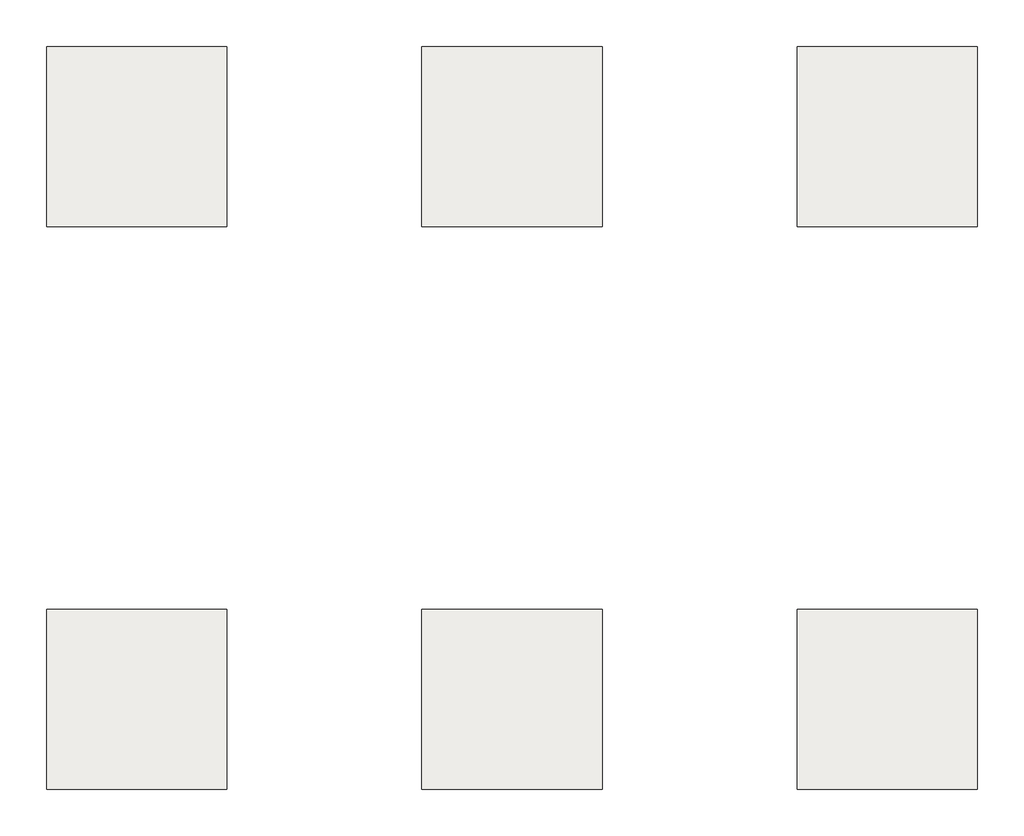
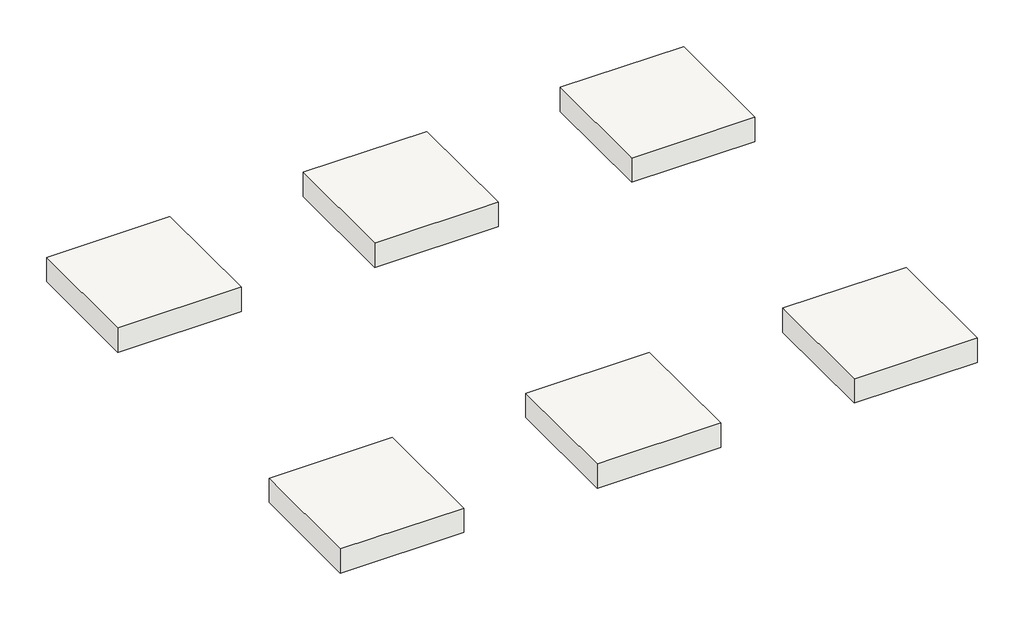
# Not in any storey: 6 slabs.
"""IFC4 building model written with IfcOpenShell, lengths in millimetres."""

import ifcopenshell
import ifcopenshell.guid

model = None  # the IFC model being written
_history = None  # IfcOwnerHistory: only IFC2X3 demands one
_inside = {}  # id of a spatial element -> (the spatial element, [elements in it])
_under = {}  # id of a project, library or spatial element -> (it, [spatial elements below it])
_declared = {}  # id of a project -> (the project, [libraries it declares])
_typed = {}  # id of a type object -> (the type object, [elements of that type])
_made_of = {}  # id of a material, layer set ... -> (it, [elements and type objects made of it])


def new_model(schema):
    """Start an empty IFC model of exactly this schema.

    Asked for "IFC4X3", IfcOpenShell would pick the latest addendum, in which some entities
    have other attributes; the version numbers below select the first issue.
    IFC2X3 requires an IfcOwnerHistory on every rooted entity: one is made here for all.
    """
    global model, _history
    if schema == "IFC4X3":
        model = ifcopenshell.file(schema_version=(4, 3, 0, 0))
    else:
        model = ifcopenshell.file(schema=schema)
    _inside.clear()
    _under.clear()
    _declared.clear()
    _typed.clear()
    _made_of.clear()
    _history = None
    if model.schema == "IFC2X3":
        org = make("IfcOrganization", Name="unknown")
        user = make(
            "IfcPersonAndOrganization",
            ThePerson=make("IfcPerson", FamilyName="unknown"),
            TheOrganization=org,
        )
        app = make(
            "IfcApplication",
            ApplicationDeveloper=org,
            Version="unknown",
            ApplicationFullName="unknown",
            ApplicationIdentifier="unknown",
        )
        _history = make(
            "IfcOwnerHistory",
            OwningUser=user,
            OwningApplication=app,
            ChangeAction="ADDED",
            CreationDate=0,
        )
    return model


def make(cls, **values):
    """One entity of the class cls with the attributes given. An attribute that is None is left unset."""
    return model.create_entity(
        cls, **{name: value for name, value in values.items() if value is not None}
    )


def rooted(cls, **values):
    """An entity with a GlobalId (a new one), such as an element, a storey or a relation."""
    return make(cls, GlobalId=ifcopenshell.guid.new(), OwnerHistory=_history, **values)


def si_unit(unit_type, name, prefix=None):
    """IfcSIUnit, for example si_unit("LENGTHUNIT", "METRE", prefix="MILLI")."""
    return make("IfcSIUnit", UnitType=unit_type, Prefix=prefix, Name=name)


def assignment(units):
    """IfcUnitAssignment: the units of a project."""
    return None if units is None else make("IfcUnitAssignment", Units=units)


def point(xyz):
    """IfcCartesianPoint."""
    return None if xyz is None else make("IfcCartesianPoint", Coordinates=xyz)


def direction(xyz):
    """IfcDirection."""
    return None if xyz is None else make("IfcDirection", DirectionRatios=xyz)


def frame(location, z_axis=None, x_axis=None):
    """IfcAxis2Placement3D, a coordinate frame: its origin and axes. An axis left out is left unset."""
    return make(
        "IfcAxis2Placement3D",
        Location=point(location),
        Axis=direction(z_axis),
        RefDirection=direction(x_axis),
    )


def origin():
    """The frame at (0, 0, 0) with its axes left unset."""
    return frame((0.0, 0.0, 0.0))


def place(relative_to, where):
    """IfcLocalPlacement: puts the frame where relative to a parent placement (None: the world)."""
    return make(
        "IfcLocalPlacement", PlacementRelTo=relative_to, RelativePlacement=where
    )


def context(
    kind, dimensions, precision=None, world=None, true_north=None, identifier=None
):
    """IfcGeometricRepresentationContext, for example the 3D "Model" context."""
    return make(
        "IfcGeometricRepresentationContext",
        ContextIdentifier=identifier,
        ContextType=kind,
        CoordinateSpaceDimension=dimensions,
        Precision=precision,
        WorldCoordinateSystem=world,
        TrueNorth=true_north,
    )


def project(units=None, contexts=None):
    """IfcProject with its units and contexts."""
    return rooted(
        "IfcProject",
        Name="project",
        RepresentationContexts=contexts,
        UnitsInContext=assignment(units),
    )


def spatial(cls, under=None, at=None, **own):
    """A site, building, storey or space (cls), placed at a placement, below another one or the project."""
    s = rooted(cls, ObjectPlacement=at, **own)
    if under is not None:
        _under.setdefault(under.id(), (under, []))[1].append(s)
    return s


def polyline(points):
    """IfcPolyline through the points."""
    return make("IfcPolyline", Points=[point(p) for p in points])


def outline(outer, holes=None, kind="AREA"):
    """IfcArbitraryClosedProfileDef: a profile drawn as a closed curve; with holes, ...WithVoids."""
    if holes is None:
        return make("IfcArbitraryClosedProfileDef", ProfileType=kind, OuterCurve=outer)
    return make(
        "IfcArbitraryProfileDefWithVoids",
        ProfileType=kind,
        OuterCurve=outer,
        InnerCurves=holes,
    )


def extrude(swept, where, along, depth):
    """IfcExtrudedAreaSolid: the profile swept, set in the frame where, extruded along a direction by depth."""
    return make(
        "IfcExtrudedAreaSolid",
        SweptArea=swept,
        Position=where,
        ExtrudedDirection=direction(along),
        Depth=depth,
    )


def shape(context_of_items, identifier, shape_type, items):
    """IfcShapeRepresentation: the items that make up one representation, for example the "Body"."""
    return make(
        "IfcShapeRepresentation",
        ContextOfItems=context_of_items,
        RepresentationIdentifier=identifier,
        RepresentationType=shape_type,
        Items=items,
    )


def source(mapping_origin, context_of_items, identifier, shape_type, items):
    """IfcRepresentationMap: a shape defined once, which mapped items show again and again."""
    return make(
        "IfcRepresentationMap",
        MappingOrigin=mapping_origin,
        MappedRepresentation=shape(context_of_items, identifier, shape_type, items),
    )


def transform(
    local_origin,
    x_axis=None,
    y_axis=None,
    z_axis=None,
    scale=None,
    scale2=None,
    scale3=None,
    uniform=True,
):
    """IfcCartesianTransformationOperator3D, or its non-uniform kind. x_axis, y_axis, z_axis: its Axis1, 2, 3."""
    if uniform:
        return make(
            "IfcCartesianTransformationOperator3D",
            Axis1=direction(x_axis),
            Axis2=direction(y_axis),
            LocalOrigin=point(local_origin),
            Scale=scale,
            Axis3=direction(z_axis),
        )
    return make(
        "IfcCartesianTransformationOperator3DnonUniform",
        Axis1=direction(x_axis),
        Axis2=direction(y_axis),
        LocalOrigin=point(local_origin),
        Scale=scale,
        Axis3=direction(z_axis),
        Scale2=scale2,
        Scale3=scale3,
    )


def mapped(mapping_source, mapping_target):
    """IfcMappedItem: shows the shape of a source again, moved by a transform."""
    return make(
        "IfcMappedItem", MappingSource=mapping_source, MappingTarget=mapping_target
    )


def made_of(thing, what):
    """Note that an element or type object is made of a material, layer set ...; save() writes the relation."""
    if what is not None:
        _made_of.setdefault(what.id(), (what, []))[1].append(thing)
    return thing


def element(
    cls,
    number,
    at=None,
    inside=None,
    cuts=None,
    type_object=None,
    material=None,
    context=None,
    identifier="Body",
    shape_type=None,
    held_by="IfcProductDefinitionShape",
    body=None,
    shapes=None,
    **own,
):
    """One element of the class cls, such as IfcWall. Its Tag is "e" and its number.

    at: its placement. inside: the storey or other place that contains it. cuts: it is an
    opening in that element (IfcRelVoidsElement). A single representation is given by context,
    identifier, shape_type and body (its items); several are given by shapes. held_by: the class
    of the entity that holds the representations. save() writes the other relations.
    """
    e = rooted(cls, Tag="e%d" % number, ObjectPlacement=at, **own)
    if body is not None:
        shapes = [shape(context, identifier, shape_type, body)]
    if shapes is not None:
        e.Representation = make(held_by, Representations=shapes)
    if inside is not None:
        _inside.setdefault(inside.id(), (inside, []))[1].append(e)
    if cuts is not None:
        rooted(
            "IfcRelVoidsElement", RelatingBuildingElement=cuts, RelatedOpeningElement=e
        )
    if type_object is not None:
        _typed.setdefault(type_object.id(), (type_object, []))[1].append(e)
    return made_of(e, material)


def aggregate(whole, parts):
    """IfcRelAggregates: a whole, such as a stair, and the parts it consists of."""
    return rooted("IfcRelAggregates", RelatingObject=whole, RelatedObjects=parts)


def save(model, path):
    """Write the relations noted so far, then the file.

    IfcRelAggregates (storeys below a building ...), IfcRelContainedInSpatialStructure (elements
    in a storey), IfcRelDefinesByType, IfcRelAssociatesMaterial and IfcRelDeclares: one each for
    every whole, place, type object, material and project.
    """
    for whole, parts in _under.values():
        aggregate(whole, parts)
    for where, things in _inside.values():
        rooted(
            "IfcRelContainedInSpatialStructure",
            RelatedElements=things,
            RelatingStructure=where,
        )
    for kind, things in _typed.values():
        rooted("IfcRelDefinesByType", RelatedObjects=things, RelatingType=kind)
    for what, things in _made_of.values():
        rooted("IfcRelAssociatesMaterial", RelatedObjects=things, RelatingMaterial=what)
    for by, libraries in _declared.values():
        rooted("IfcRelDeclares", RelatingContext=by, RelatedDefinitions=libraries)
    model.write(path)


def ft211_2400x2400x500_5fe39465(model_context):
    return source(origin(), model_context, "Body", "SweptSolid", [
        extrude(outline(polyline([(1200.0, 1200.0), (1200.0, -1200.0), (-1200.0, -1200.0), (-1200.0, 1200.0), (1200.0, 1200.0)])), frame((0.0, 0.0, -500.0), z_axis=(0.0, 0.0, 1.0), x_axis=(1.0, 0.0, 0.0)), (0.0, 0.0, 1.0), 500.0),
    ])


model = new_model("IFC4")

# Units and contexts
model_context = context("Model", 3, world=origin())
ifc_project = project(units=[si_unit("LENGTHUNIT", "METRE", prefix="MILLI")], contexts=[model_context])

# Site, building
site = spatial("IfcSite", under=ifc_project)
building = spatial("IfcBuilding", under=site)

# Slabs
placement = place(None, origin())
element("IfcSlab", 1, ObjectType="FT211-Footing-Rectangular_더미삭제 : FT211_2400x2400x500", at=placement, inside=building, context=model_context, shape_type="SweptSolid", body=[
    extrude(outline(polyline([(11200.0, 22199.5208589), (11200.0, 19799.5208589), (8800.0, 19799.5208589), (8800.0, 22199.5208589), (11200.0, 22199.5208589)])), frame((0.0, 0.0, -1800.0), z_axis=(0.0, 0.0, 1.0), x_axis=(1.0, 0.0, 0.0)), (0.0, 0.0, 1.0), 500.0),
])
element("IfcSlab", 2, ObjectType="FT211-Footing-Rectangular_더미삭제 : FT211_2400x2400x500", at=placement, inside=building, context=model_context, shape_type="SweptSolid", body=[
    extrude(outline(polyline([(6200.0, 22199.5208589), (6200.0, 19799.5208589), (3800.0, 19799.5208589), (3800.0, 22199.5208589), (6200.0, 22199.5208589)])), frame((0.0, 0.0, -1800.0), z_axis=(0.0, 0.0, 1.0), x_axis=(1.0, 0.0, 0.0)), (0.0, 0.0, 1.0), 500.0),
])
element("IfcSlab", 3, ObjectType="FT211-Footing-Rectangular_더미삭제 : FT211_2400x2400x500", at=placement, inside=building, context=model_context, shape_type="SweptSolid", body=[
    extrude(outline(polyline([(1200.0, 22199.5208589), (1200.0, 19799.5208589), (-1200.0, 19799.5208589), (-1200.0, 22199.5208589), (1200.0, 22199.5208589)])), frame((0.0, 0.0, -1800.0), z_axis=(0.0, 0.0, 1.0), x_axis=(1.0, 0.0, 0.0)), (0.0, 0.0, 1.0), 500.0),
])
element("IfcSlab", 4, ObjectType="FT211-Footing-Rectangular_더미삭제 : FT211_2400x2400x500", at=placement, inside=building, context=model_context, shape_type="SweptSolid", body=[
    extrude(outline(polyline([(1200.0, 14699.5208589), (1200.0, 12299.5208589), (-1200.0, 12299.5208589), (-1200.0, 14699.5208589), (1200.0, 14699.5208589)])), frame((0.0, 0.0, -1800.0), z_axis=(0.0, 0.0, 1.0), x_axis=(1.0, 0.0, 0.0)), (0.0, 0.0, 1.0), 500.0),
])
ft211_2400x2400x500_shape = ft211_2400x2400x500_5fe39465(model_context)
element("IfcSlab", 5, ObjectType="FT211-Footing-Rectangular_더미삭제 : FT211_2400x2400x500", at=placement, inside=building, context=model_context, shape_type="MappedRepresentation", body=[
    mapped(ft211_2400x2400x500_shape, transform((5000.0, 13499.5208589, -1300.0), x_axis=(1.0, 0.0, 0.0), y_axis=(0.0, 1.0, 0.0), z_axis=(0.0, 0.0, 1.0))),
])
element("IfcSlab", 6, ObjectType="FT211-Footing-Rectangular_더미삭제 : FT211_2400x2400x500", at=placement, inside=building, context=model_context, shape_type="MappedRepresentation", body=[
    mapped(ft211_2400x2400x500_shape, transform((10000.0, 13499.5208589, -1300.0), x_axis=(1.0, 0.0, 0.0), y_axis=(0.0, 1.0, 0.0), z_axis=(0.0, 0.0, 1.0))),
])

save(model, "model.ifc")

# Revit data of these elements
# Project information
#   Building Name = "MAIN GATE SECURITY BUILDING"
#   Project Status = "Project Status"
#   Client Name = "현대엔지니어링"
#   Project Address = "서울시 종로구 율곡로 75(계동)"
#   Project Name = "Therma Visayas Energy Project"
#   Project Number = "-"
# Grids (mm)
#   "A": line (0, 24502.793) -> (0, 11308.625)
#   "B": line (5000, 24502.793) -> (5000, 11308.625)
#   "C": line (10000, 24502.793) -> (10000, 11308.625)
#   "1": line (-3860.098, 13499.521) -> (12441.468, 13499.521)
#   "2": line (-3860.098, 20999.521) -> (12441.468, 20999.521)
# Type "FT211-Footing-Rectangular_더미삭제 : FT211_2400x2400x500"
#   Top bar = "D25@300"
#   Description = "UG Shallow Foundation"
#   Bottom bar = "D20@300"
#   Width = 2400 mm
#   Length = 2400 mm
#   Foundation Thickness = 500 mm
#   Structural Material [instance default] = A03AC032-00007_Structural Concrete_Type1_25MPa-30Mpa
#   Assembly Code = ""
# Elements 1, 2, 3, 4, 5, 6 (IfcSlab, "FT211-Footing-Rectangular_더미삭제 : FT211_2400x2400x500")
#   Comments = ""
#   Mark = "F1"
#   F01) Building Name = "Main Gate House"
#   F11) Project Building Tag_Type-1 = "Common"
#   F12) Project Building Tag_Type-2 = "Common"
#   F13) Project Facility Code = "Facility Code"
#   F21) Structural Type = "Concrete"
#   F31) Standard Building Code = "IBC"
#   F41) Discipline = "AR"
#   F51) Plan Start Date-Engineering = "2015-01-01"
#   F52) Plan Finish Date-Engineering = "2015-12-31"
#   F53) Duration = "365"
#   F54) Actual Start Date-Engineering = "2015-01-01"
#   F55) Actual Finish Date-Engineering = "2015-12-31"
#   F61) Plan Start Date-Construction = "2016-08-19"
#   F62) Plan Finish Date-Construction = "2017-01-31"
#   F64) Actual Start Date-Construction = "2016-08-19"
#   F63) Duration = "202"
#   F65) Actual Finish Date-Construction = "2017-01-31"
#   F91) Plant Type = "CFPP"
#   F92) KKS Structures, Building = "UYF"
#   P01) Project Name = "TVEP"
#   P02) Project Configuration = "CFB Boiler x 2(Foster Wheeler) + STG x 2(Alstom, 150MW)"
#   P03) Project Abbreviation = "TVEP"
#   P04) Project Code = "BEPH1402"
#   P05) Project Stage = "In operation"
#   P06) Project Location = "Sito Looc, Barangay Bato, Toledo City in Philippines"
#   P07) Project Owner = "Therma Visayas, Inc."
#   P08) Project O.E = "Flour"
#   P09) Project Schedule = "ITB Issueing Date : 2013.07.30\r\nSite Survey : 2013.08.19-20\r\nBid Closing Date : 2013.11.29\r\nPreferred Bidder Notice 접수 : 2014.04.27\r\nTarget award date : 2014 05\r\nLOA 접수 : 2014.05.21\r\nSigning Ceremony : 2014.05.30"
#   P10) Basic Wind Speed = "55.6 m/s"
#   P11) Seismic = "NSCP 2010, Zone 4 (PGA : 0.4g)"
#   P12) Soil = "Sc"
#   P13) Soil Capacity = "100kN/m2"
#   P14) Pile Capacity = "PHC(D400) : 1200kN"
#   W00) Work Master Code = "A03AC032-00007"
#   W01) Work Master_Lv1 = "Concrete Work"
#   W02) Work Master_Lv2 = "Substructure Work"
#   W03) Work Master_Spec.1 = "Cement Type-1"
#   W04) Work Master_Spec.2 = "25MPa < F'c (Cylinder Strength) ≤ 30MPa"
#   W11) Activity ID = "C02AGB010"
#   W12) Activity Name = "Main Gate Security Building - Building Foundation"
#   W13) Plan Start Date = "2016-08-19"
#   W14) Plan Finish Date = "2016-09-22"
#   W15) Duration = "26"
#   W16) Actual Start Date = "2016-08-19"
#   W17) Actual Finish Date = "2016-09-22"
#   R02) Unit Price = 0
#   Structural Material = A03AC032-00007_Structural Concrete_Type1_25MPa-30Mpa
#   Phase Created = New Construction
#   Materials on its faces: "A03AC032-00007_Structural Concrete_Type1_25MPa-30Mpa"
# Materials
#   "A03AC032-00007_Structural Concrete_Type1_25MPa-30Mpa": class "Concrete", colour RGB 176 176 176, transparency 0, Keynote = "09910.A1", Description = "Reinf. Conc.", W00) Work Master Code = "A03AC032-00007", W01) Work Master_Lv1 = "Concrete Work", W02) Work Master_Lv2 = "Substructure Work", W03) Work Master_Spec.1 = "Structural Concrete", W04) Work Master_Spec.2 = "Cement Type-1", W05) Work Master_Spec.3 = "25MPa < F'c (Cylinder Strength) ≤ 30MPa", Cost = 0
